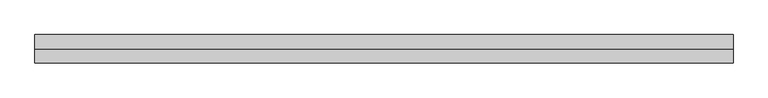
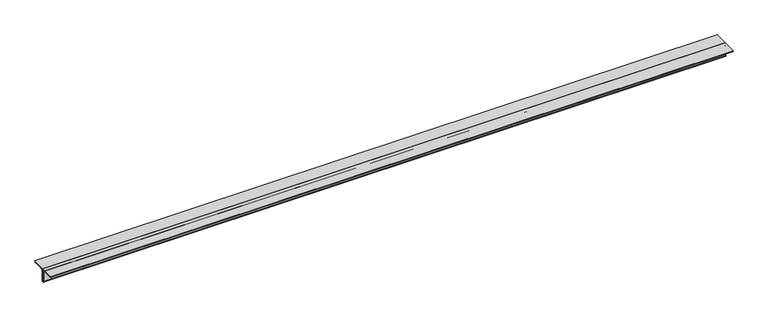
"""IFC4 building model written with IfcOpenShell, lengths in millimetres: member geometry, Steel Framing_2Ls_KS : H_SB_AR_S02_2Ls-100x100x10_VBR1."""

from ifc_helpers import new_model, si_unit, point, frame, frame_2d, origin, place, context, project, spatial, polyline, circle_curve, trimmed, segment, composite_curve, outline, extrude, source, transform, mapped, element, save


def member_e2534760(model_context):
    return source(origin(), model_context, "Body", "SweptSolid", [
        extrude(outline(composite_curve([segment(polyline([(0.0, 28.2), (100.0, 28.2)]), True, "CONTINUOUS"), segment(trimmed(circle_curve(frame_2d((90.0, 28.2)), 10.0), [point((100.0, 28.2))], [point((90.0, 18.2))], False, "CARTESIAN"), True, "CONTINUOUS"), segment(polyline([(90.0, 18.2), (20.0, 18.2)]), True, "CONTINUOUS"), segment(trimmed(circle_curve(frame_2d((20.0, 8.2)), 10.0), [point((20.0, 18.2))], [point((10.0, 8.2))], True, "CARTESIAN"), True, "CONTINUOUS"), segment(polyline([(10.0, 8.2), (10.0, -61.8)]), True, "CONTINUOUS"), segment(trimmed(circle_curve(frame_2d((0.0, -61.8)), 10.0), [point((10.0, -61.8))], [point((0.0, -71.8))], False, "CARTESIAN"), True, "CONTINUOUS"), segment(polyline([(0.0, -71.8), (0.0, 28.2)]), True, "CONTINUOUS")], self_intersect=False)), frame((-2590.3354834, 0.0, 0.0), z_axis=(1.0, 0.0, 0.0), x_axis=(0.0, 1.0, 0.0)), (0.0, 0.0, 1.0), 4915.1757569),
        extrude(outline(composite_curve([segment(polyline([(0.0, 28.2), (0.0, -71.8)]), True, "CONTINUOUS"), segment(trimmed(circle_curve(frame_2d((0.0, -61.8)), 10.0), [point((0.0, -71.8))], [point((-10.0, -61.8))], False, "CARTESIAN"), True, "CONTINUOUS"), segment(polyline([(-10.0, -61.8), (-10.0, 8.2)]), True, "CONTINUOUS"), segment(trimmed(circle_curve(frame_2d((-20.0, 8.2)), 10.0), [point((-10.0, 8.2))], [point((-20.0, 18.2))], True, "CARTESIAN"), True, "CONTINUOUS"), segment(polyline([(-20.0, 18.2), (-90.0, 18.2)]), True, "CONTINUOUS"), segment(trimmed(circle_curve(frame_2d((-90.0, 28.2)), 10.0), [point((-90.0, 18.2))], [point((-100.0, 28.2))], False, "CARTESIAN"), True, "CONTINUOUS"), segment(polyline([(-100.0, 28.2), (0.0, 28.2)]), True, "CONTINUOUS")], self_intersect=False)), frame((-2590.3354834, 0.0, 0.0), z_axis=(1.0, 0.0, 0.0), x_axis=(0.0, 1.0, 0.0)), (0.0, 0.0, 1.0), 4915.1757569),
    ])


if __name__ == "__main__":
    model = new_model("IFC4")
    model_context = context("Model", 3, world=origin())
    ifc_project = project(units=[si_unit("LENGTHUNIT", "METRE", prefix="MILLI")], contexts=[model_context])
    site = spatial("IfcSite", under=ifc_project)
    building = spatial("IfcBuilding", under=site)
    placement = place(None, origin())
    member_shape = member_e2534760(model_context)
    element("IfcMember", 1, ObjectType="Steel Framing_2Ls_KS : H_SB_AR_S02_2Ls-100x100x10_VBR1", at=placement, inside=building, context=model_context, shape_type="MappedRepresentation", body=[
        mapped(member_shape, transform((0.0, 0.0, 0.0), x_axis=(1.0, 0.0, 0.0), y_axis=(0.0, 1.0, 0.0), z_axis=(0.0, 0.0, 1.0))),
    ])
    save(model, "model.ifc")

# Revit data of these elements
# Type "Steel Framing_2Ls_KS : H_SB_AR_S02_2Ls-100x100x10_VBR1"
#   Type Comments = "MAIN"
#   Type Mark = "VBR1"
#   H_SectionID = "2Ls-100x100x10"
#   Assembly Code = "B10"
#   Legs = "LLBB"
#   H_Ratio for Additional Steel Plate = 0.2
#   W = 0
#   Perimeter = 0.80 m²/m
#   Nominal Weight = 29.80 kgf/m
#   Length [instance default] = 1524 mm
#   Space = 0 mm
#   b = 100 mm
#   d = 100 mm
#   t = 10 mm
#   y = 28.2 mm
#   A = 0.0038 m²
#   Structural Material [instance default] = Steel, 45-345
# Element 1 (IfcMember, "Steel Framing_2Ls_KS : H_SB_AR_S02_2Ls-100x100x10_VBR1")
#   Materials on its faces: "Steel, 45-345"
# Materials
#   "Steel, 45-345": class "Metal", colour RGB 189 187 185, transparency 0, Description = "Steel 345 MPa", Cost = 0
